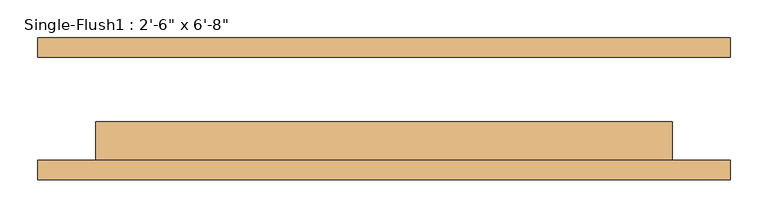
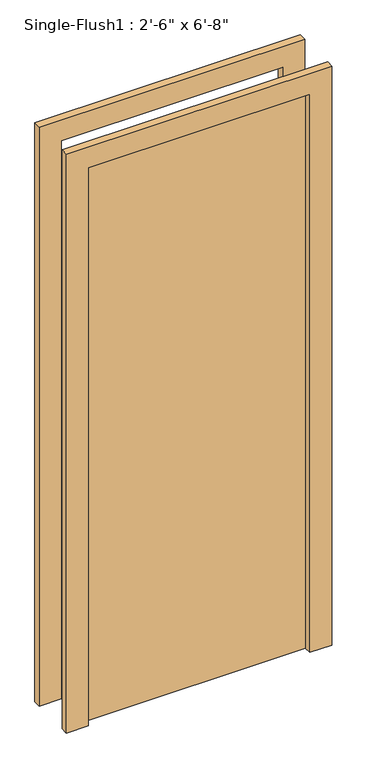
"""IFC4 building model written with IfcOpenShell, lengths in millimetres: door geometry."""

from ifc_helpers import new_model, si_unit, frame, origin, origin_with_axes, place, context, project, spatial, polyline, outline, extrude, source, transform, mapped, element, save


def door_cf295576(model_context):
    return source(origin(), model_context, "Body", "SweptSolid", [
        extrude(outline(polyline([(2108.2, -457.2), (0.0, -457.2), (0.0, -381.0), (2032.0, -381.0), (2032.0, 381.0), (0.0, 381.0), (0.0, 457.2), (2108.2, 457.2), (2108.2, -457.2)])), frame((0.0, -93.6625, 0.0), z_axis=(0.0, 1.0, 0.0), x_axis=(0.0, 0.0, 1.0)), (0.0, 0.0, 1.0), 25.4),
        extrude(outline(polyline([(2108.2, 457.2), (2108.2, -457.2), (0.0, -457.2), (0.0, -381.0), (2032.0, -381.0), (2032.0, 381.0), (0.0, 381.0), (0.0, 457.2), (2108.2, 457.2)])), frame((0.0, 68.2625, 0.0), z_axis=(0.0, 1.0, 0.0), x_axis=(0.0, 0.0, 1.0)), (0.0, 0.0, 1.0), 25.4),
        extrude(outline(polyline([(381.0, -17.4625), (381.0, -68.2625), (-381.0, -68.2625), (-381.0, -17.4625), (381.0, -17.4625)])), origin_with_axes(), (0.0, 0.0, 1.0), 2032.0),
    ])


if __name__ == "__main__":
    model = new_model("IFC4")
    model_context = context("Model", 3, world=origin())
    ifc_project = project(units=[si_unit("LENGTHUNIT", "METRE", prefix="MILLI")], contexts=[model_context])
    site = spatial("IfcSite", under=ifc_project)
    building = spatial("IfcBuilding", under=site)
    placement = place(None, origin())
    door_shape = door_cf295576(model_context)
    element("IfcDoor", 1, ObjectType="Single-Flush1 : 2'-6\" x 6'-8\"", at=placement, inside=building, context=model_context, shape_type="MappedRepresentation", body=[
        mapped(door_shape, transform((0.0, 0.0, 0.0), x_axis=(1.0, 0.0, 0.0), y_axis=(0.0, 1.0, 0.0), z_axis=(0.0, 0.0, 1.0))),
    ])
    save(model, "model.ifc")

# Revit data of these elements
# Type "Single-Flush1 : 2'-6\" x 6'-8\""
#   Type Mark = "25"
#   Construction Type Id = "MDOOR"
#   Assembly Code = "C1020"
#   Analytic Construction = "Metal"
#   Thickness = 0' - 2"
#   Heat Transfer Coefficient (U) = 3.7021 W/(m²·K)
#   Height = 6' - 8"
#   Trim Projection Ext = 0' - 1"
#   Trim Projection Int = 0' - 1"
#   Trim Width = 0' - 3"
#   Width = 2' - 6"
#   Door Material = Door - Panel
#   Frame Material = Door - Frame
#   Visual Light Transmittance = 0
#   Solar Heat Gain Coefficient = 0
#   Function = (empty or 0)
#   Wall Closure = (empty or 0)
# Element 1 (IfcDoor, "Single-Flush1 : 2'-6\" x 6'-8\"")
#   Materials on its faces: "Door - Frame", "Door - Panel"
# Materials
#   "Door - Panel": class "Wood", colour RGB 210 159 95, transparency 0, Cost = 0
#   "Door - Frame": class "Miscellaneous", colour RGB 118 70 51, transparency 0, Cost = 0
